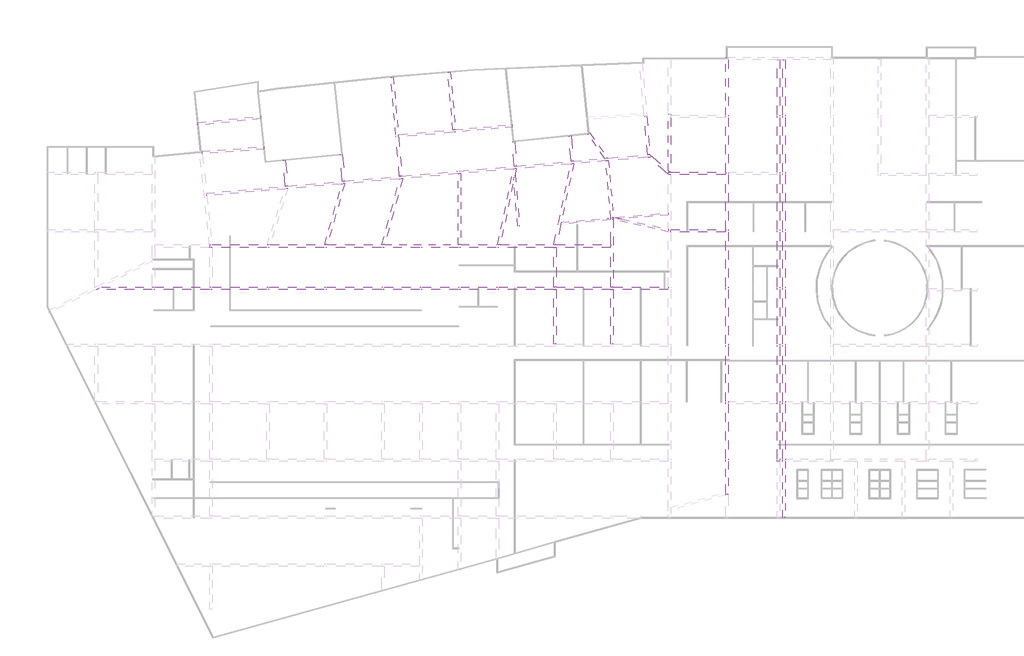
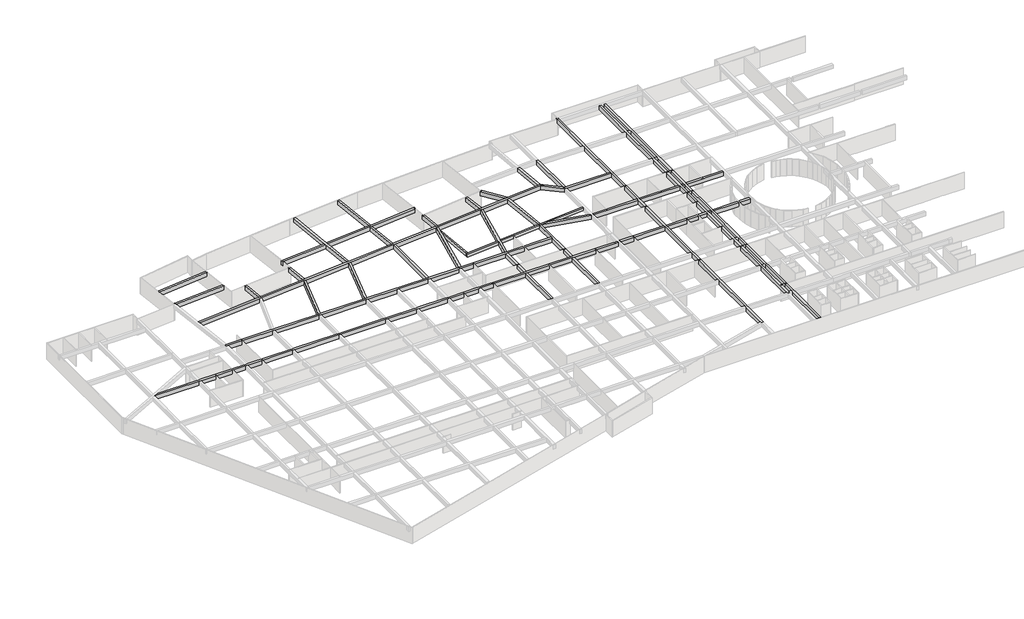
# One storey, part 7 of 8: 34 beams.
# Revit data of these elements (continued)
# Type "混凝土 - 矩形梁 : KL_beam"
#   Length [instance default] = 1524 mm
#   b = 400 mm
#   h = 800 mm
#   Structural Material [instance default] = 混凝土 - 现场浇注混凝土
#   Assembly Code = ""
# Type "混凝土 - 矩形梁 : L_beam"
#   Length [instance default] = 1524 mm
#   b = 300 mm
#   h = 600 mm
#   Structural Material [instance default] = none
#   Assembly Code = ""
# Elements 1, 2, 3, 4, 5, 6, 7, 8, 9, 10, 11, 12, 13, 14, 15, 16, 17, 18, 19, 20, 21, 22, 23, 24, 25, 26, 27, 28, 29, 30, 31, 32 (IfcBeam, "混凝土 - 矩形梁 : KL_beam")
#   Comments = ""
#   Structural Material = none
#   Phase Created = 新构造
# Elements 33, 34 (IfcBeam, "混凝土 - 矩形梁 : L_beam")
#   Comments = ""
#   Structural Material = none
#   Phase Created = 新构造
# Materials
#   "混凝土 - 现场浇注混凝土": class "混凝土", colour RGB 192 192 192, transparency 0
